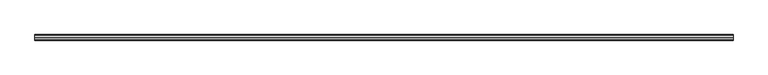
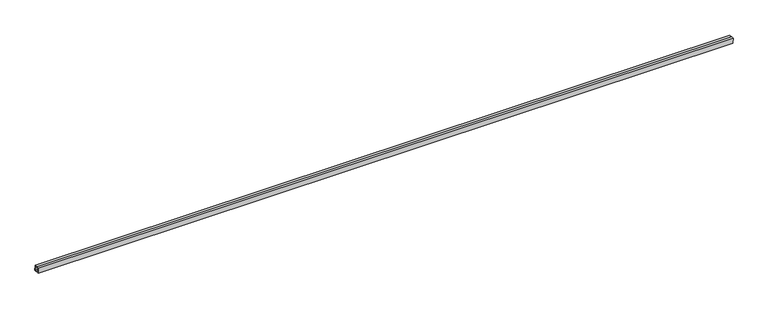
"""IFC4 building model written with IfcOpenShell, lengths in millimetres: proxy geometry, Inner panel:Inner panel:1:Inner panel:1 : Inner panel:Inner panel:300324:2:Inner panel:1:Inner panel:1 : Inner panel:Inner panel:300324:2 : Inner panel:Inner panel:1:Inner panel:1 : Inner panel:Inner panel:300324:300043:25 : Inner panel:Inner panel:1:Inner panel:1 : Inner panel:Inner panel:300324:2:Inner panel:1:Inner panel:1 : Inner panel:Inner panel:300324:2 : Inner panel:Inner panel:1:Inner panel:1 : Inner panel:Inner panel:300324:300043:308120."""

from ifc_helpers import new_model, si_unit, frame, origin, place, context, project, spatial, polyline, outline, extrude, source, transform, mapped, element, save


def generic_models_b7d1631c(model_context):
    return source(origin(), model_context, "Body", "SweptSolid", [
        extrude(outline(polyline([(-569061.6758054, 8767.2361869), (-569043.4353822, 8767.9962045), (-569041.8492584, 8729.9292345), (-569079.9162285, 8728.3431107), (-569081.5023523, 8766.4100808), (-569063.2619291, 8767.1700984), (-569063.1627964, 8764.7909128), (-569079.0240339, 8764.1300279), (-569077.6361756, 8730.8214291), (-569044.3275768, 8732.2092874), (-569045.7154351, 8765.5178862), (-569061.5766726, 8764.8570013), (-569061.6758054, 8767.2361869)])), frame((588245.3367242, 0.0, 0.0), z_axis=(1.0, 0.0, 0.0), x_axis=(0.0, 1.0, 0.0)), (0.0, 0.0, 1.0), 4876.8),
    ])


if __name__ == "__main__":
    model = new_model("IFC4")
    model_context = context("Model", 3, world=origin())
    ifc_project = project(units=[si_unit("LENGTHUNIT", "METRE", prefix="MILLI")], contexts=[model_context])
    site = spatial("IfcSite", under=ifc_project)
    building = spatial("IfcBuilding", under=site)
    placement = place(None, origin())
    generic_models_shape = generic_models_b7d1631c(model_context)
    element("IfcBuildingElementProxy", 1, Name="Inner panel:Inner panel:1:Inner panel:1 : Inner panel:Inner panel:300324:2:Inner panel:1:Inner panel:1 : Inner panel:Inner panel:300324:2 : Inner panel:Inner panel:1:Inner panel:1 : Inner panel:Inner panel:300324:300043:25 : Inner panel:Inner panel:1:Inner panel:1 : Inner panel:Inner panel:300324:2:Inner panel:1:Inner panel:1 : Inner panel:Inner panel:300324:2 : Inner panel:Inner panel:1:Inner panel:1 : Inner panel:Inner panel:300324:300043:308120", ObjectType="Inner panel:Inner panel:1:Inner panel:1 : Inner panel:Inner panel:300324:2:Inner panel:1:Inner panel:1 : Inner panel:Inner panel:300324:2 : Inner panel:Inner panel:1:Inner panel:1 : Inner panel:Inner panel:300324:300043:25 : Inner panel:Inner panel:1:Inner panel:1 : Inner panel:Inner panel:300324:2:Inner panel:1:Inner panel:1 : Inner panel:Inner panel:300324:2 : Inner panel:Inner panel:1:Inner panel:1 : Inner panel:Inner panel:300324:300043:308120", at=placement, inside=building, context=model_context, shape_type="MappedRepresentation", body=[
        mapped(generic_models_shape, transform((0.0, 0.0, 0.0), x_axis=(1.0, 0.0, 0.0), y_axis=(0.0, 1.0, 0.0), z_axis=(0.0, 0.0, 1.0))),
    ])
    save(model, "model.ifc")

# Revit data of these elements
# Type "Inner panel:Inner panel:1:Inner panel:1 : Inner panel:Inner panel:300324:2:Inner panel:1:Inner panel:1 : Inner panel:Inner panel:300324:2 : Inner panel:Inner panel:1:Inner panel:1 : Inner panel:Inner panel:300324:300043:25 : Inner panel:Inner panel:1:Inner panel:1 : Inner panel:Inner panel:300324:2:Inner panel:1:Inner panel:1 : Inner panel:Inner panel:300324:2 : Inner panel:Inner panel:1:Inner panel:1 : Inner panel:Inner panel:300324:300043:308120"
#   NameOverride = "Inner panel:Inner panel:1:Inner panel:1 : Inner panel:Inner panel:300324:2:Inner panel:1:Inner panel:1 : Inner panel:Inner panel:300324:2 : Inner panel:Inner panel:1:Inner panel:1 : Inner panel:Inner panel:300324:300043:308120"
#   ObjectTypeOverride = "Inner panel:1:Inner panel:1 : Inner panel:Inner panel:300324:2 : Inner panel:Inner panel:1:Inner panel:1 : Inner panel:Inner panel:300324:300043"
#   Reference = "Inner panel"
#   Tag = "308120"
# Element 1 (IfcBuildingElementProxy, "Inner panel:Inner panel:1:Inner panel:1 : Inner panel:Inner panel:300324:2:Inner panel:1:Inner panel:1 : Inner panel:Inner panel:300324:2 : Inner panel:Inner panel:1:Inner panel:1 : Inner panel:Inner panel:300324:300043:25 : Inner panel:Inner panel:1:Inner panel:1 : Inner panel:Inner panel:300324:2:Inner panel:1:Inner panel:1 : Inner panel:Inner panel:300324:2 : Inner panel:Inner panel:1:Inner panel:1 : Inner panel:Inner panel:300324:300043:308120")
#   Materials on its faces: "1 1/2\" X 1 1/2\" SPLIT-SEAM SQUARE TUBING (~24\" CANTILEVER FROM C.L. OF GLULAM)"
# Materials
#   "1 1/2\" X 1 1/2\" SPLIT-SEAM SQUARE TUBING (~24\" CANTILEVER FROM C.L. OF GLULAM)": class "Unassigned", colour RGB 202 201 200, transparency 0, Cost = 0
